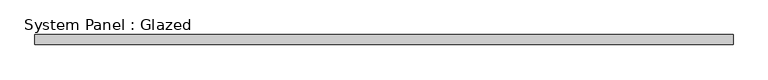
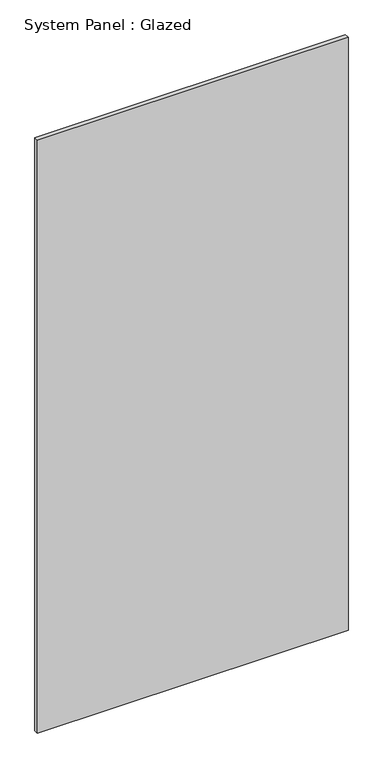
"""IFC4 building model written with IfcOpenShell, lengths in millimetres: plate geometry, System Panel : Glazed."""

from ifc_helpers import new_model, si_unit, origin, origin_with_axes, place, context, project, spatial, polyline, outline, extrude, source, transform, mapped, element, save


def system_panel_glazed_7e716341(model_context):
    return source(origin(), model_context, "Body", "SweptSolid", [
        extrude(outline(polyline([(882.65, 19.05), (-882.65, 19.05), (-882.65, 44.45), (882.65, 44.45), (882.65, 19.05)])), origin_with_axes(), (0.0, 0.0, 1.0), 3562.35),
    ])


if __name__ == "__main__":
    model = new_model("IFC4")
    model_context = context("Model", 3, world=origin())
    ifc_project = project(units=[si_unit("LENGTHUNIT", "METRE", prefix="MILLI")], contexts=[model_context])
    site = spatial("IfcSite", under=ifc_project)
    building = spatial("IfcBuilding", under=site)
    placement = place(None, origin())
    system_panel_glazed_shape = system_panel_glazed_7e716341(model_context)
    element("IfcPlate", 1, ObjectType="System Panel : Glazed", at=placement, inside=building, context=model_context, shape_type="MappedRepresentation", body=[
        mapped(system_panel_glazed_shape, transform((0.0, 0.0, 0.0), x_axis=(1.0, 0.0, 0.0), y_axis=(0.0, 1.0, 0.0), z_axis=(0.0, 0.0, 1.0))),
    ])
    save(model, "model.ifc")

# Revit data of these elements
# Type "System Panel : Glazed"
#   Construction Type Id = "GSP4R"
#   Analytic Construction = "1/8 in Pilkington single glazing"
#   Visual Light Transmittance = 0.9
#   Solar Heat Gain Coefficient = 0.86
#   Heat Transfer Coefficient (U) = 1.18115 BTU/(h·ft²·°F)
#   Define Thermal Properties by = 1
# Element 1 (IfcPlate, "System Panel : Glazed")
#   Materials on its faces: "Glass"
# Materials
#   "Glass": class "Glass", colour RGB 0 128 192, transparency 0.75, Description = "Soda Lime Glass", Cost = 0
